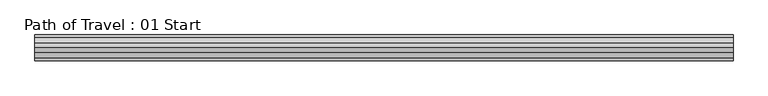
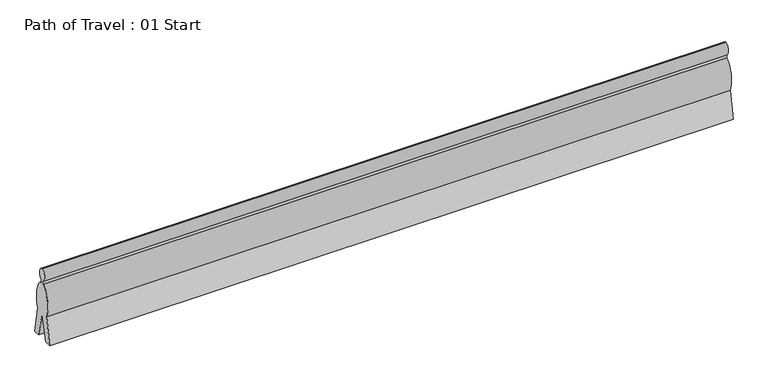
"""IFC4 building model written with IfcOpenShell, lengths in millimetres: proxy geometry, Path of Travel : 01 Start."""

from ifc_helpers import new_model, si_unit, point, frame, origin, place, context, project, spatial, ellipse_curve, trimmed, source, transform, mapped, element, save
from ifc_brep_helpers import plane_surface, extruded_surface, advanced_brep


def path_of_travel_01_start_60fd2745(model_context):
    return source(origin(), model_context, "Body", "AdvancedBrep", [
        advanced_brep(
        [(227.5554837, 0.0, 1727.2), (227.5554837, 42.9018657, 1436.6534209), (227.5554837, 42.9018657, 1363.4763406), (227.5554837, 184.1186263, 643.4144547), (227.5554837, 297.5699544, 0.0), (227.5554837, 145.6574193, 0.0), (227.5554837, 0.0, 584.2), (227.5554837, -145.6574193, 0.0), (227.5554837, -297.5699544, 0.0), (227.5554837, -184.1186263, 643.4144547), (227.5554837, -42.9018657, 1363.4763406), (227.5554837, -42.9018657, 1436.6534209), (16229.5554837, 0.0, 1727.2), (16229.5554837, -42.9018657, 1436.6534209), (16229.5554837, -42.9018657, 1363.4763406), (16229.5554837, -184.1186263, 643.4144547), (16229.5554837, -297.5699544, 0.0), (16229.5554837, -145.6574193, 0.0), (16229.5554837, 0.0, 584.2), (16229.5554837, 145.6574193, 0.0), (16229.5554837, 297.5699544, 0.0), (16229.5554837, 184.1186263, 643.4144547), (16229.5554837, 42.9018657, 1363.4763406), (16229.5554837, 42.9018657, 1436.6534209)],
        [
            (0, 1, ellipse_curve(frame((227.5554837, 0.0, 1574.8), z_axis=(-1.0, 0.0, 0.0), x_axis=(0.0, 0.0, 1.0)), 152.4, 101.6)),
            (1, 2),
            (2, 3, ellipse_curve(frame((227.5554837, 0.0, 914.4), z_axis=(-1.0, 0.0, 0.0), x_axis=(0.0, 0.0, -1.0)), 457.2, 228.6)),
            (3, 4),
            (4, 5),
            (5, 6),
            (6, 7),
            (7, 8),
            (8, 9),
            (9, 10, ellipse_curve(frame((227.5554837, 0.0, 914.4), z_axis=(-1.0, 0.0, 0.0), x_axis=(0.0, 0.0, -1.0)), 457.2, 228.6)),
            (10, 11),
            (11, 0, ellipse_curve(frame((227.5554837, 0.0, 1574.8), z_axis=(-1.0, 0.0, 0.0), x_axis=(0.0, 0.0, 1.0)), 152.4, 101.6)),
            (12, 13, ellipse_curve(frame((16229.5554837, 0.0, 1574.8), z_axis=(1.0, 0.0, 0.0), x_axis=(0.0, 0.0, 1.0)), 152.4, 101.6)),
            (13, 14),
            (14, 15, ellipse_curve(frame((16229.5554837, 0.0, 914.4), z_axis=(1.0, 0.0, 0.0), x_axis=(0.0, 0.0, -1.0)), 457.2, 228.6)),
            (15, 16),
            (16, 17),
            (17, 18),
            (18, 19),
            (19, 20),
            (20, 21),
            (21, 22, ellipse_curve(frame((16229.5554837, 0.0, 914.4), z_axis=(1.0, 0.0, 0.0), x_axis=(0.0, 0.0, -1.0)), 457.2, 228.6)),
            (22, 23),
            (23, 12, ellipse_curve(frame((16229.5554837, 0.0, 1574.8), z_axis=(1.0, 0.0, 0.0), x_axis=(0.0, 0.0, 1.0)), 152.4, 101.6)),
            (0, 12),
            (23, 1),
            (22, 2),
            (21, 3),
            (20, 4),
            (19, 5),
            (18, 6),
            (17, 7),
            (16, 8),
            (15, 9),
            (14, 10),
            (13, 11),
        ],
        [
            plane_surface(frame((227.5554837, 0.0, 0.0), z_axis=(-1.0, 0.0, 0.0), x_axis=(0.0, 0.0, 1.0))),
            plane_surface(frame((16229.5554837, 0.0, 0.0), z_axis=(1.0, 0.0, 0.0), x_axis=(0.0, 0.0, 1.0))),
            extruded_surface(trimmed(ellipse_curve(frame((16229.5554837, 0.0, 1574.8), z_axis=(-1.0, 0.0, 0.0), x_axis=(0.0, 0.0, 1.0)), 152.4, 101.6), [point((16229.5554837, 0.0, 1727.2))], [point((16229.5554837, 42.9018657, 1436.6534209))], True, "CARTESIAN"), (-16002.0, 0.0, 0.0), 16002.0),
            plane_surface(frame((227.5554837, 42.9018657, 1436.6534209), z_axis=(0.0, 1.0, 0.0), x_axis=(1.0, 0.0, 0.0))),
            extruded_surface(trimmed(ellipse_curve(frame((16229.5554837, 0.0, 914.4), z_axis=(-1.0, 0.0, 0.0), x_axis=(0.0, 0.0, -1.0)), 457.2, 228.6), [point((16229.5554837, 42.9018657, 1363.4763406))], [point((16229.5554837, 184.1186263, 643.4144547))], True, "CARTESIAN"), (-16002.0, 0.0, 0.0), 16002.0),
            plane_surface(frame((227.5554837, 184.1186263, 643.4144547), z_axis=(0.0, 0.9848077530122078, 0.17364817766693205), x_axis=(1.0, 0.0, 0.0))),
            plane_surface(frame((227.5554837, 297.5699544, 0.0), z_axis=(0.0, 0.0, -1.0), x_axis=(1.0, 0.0, 0.0))),
            plane_surface(frame((227.5554837, 145.6574193, 0.0), z_axis=(0.0, -0.9702957262760199, -0.2419218955995739), x_axis=(1.0, 0.0, 0.0))),
            plane_surface(frame((227.5554837, 0.0, 584.2), z_axis=(0.0, 0.9702957262759961, -0.24192189559966923), x_axis=(1.0, 0.0, 0.0))),
            plane_surface(frame((227.5554837, -145.6574193, 0.0), z_axis=(0.0, 0.0, -1.0), x_axis=(1.0, 0.0, 0.0))),
            plane_surface(frame((227.5554837, -297.5699544, 0.0), z_axis=(0.0, -0.984807753012208, 0.17364817766693066), x_axis=(1.0, 0.0, 0.0))),
            extruded_surface(trimmed(ellipse_curve(frame((16229.5554837, 0.0, 914.4), z_axis=(-1.0, 0.0, 0.0), x_axis=(0.0, 0.0, -1.0)), 457.2, 228.6), [point((16229.5554837, -184.1186263, 643.4144547))], [point((16229.5554837, -42.9018657, 1363.4763406))], True, "CARTESIAN"), (-16002.0, 0.0, 0.0), 16002.0),
            plane_surface(frame((227.5554837, -42.9018657, 1363.4763406), z_axis=(0.0, -1.0, 0.0), x_axis=(1.0, 0.0, 0.0))),
            extruded_surface(trimmed(ellipse_curve(frame((16229.5554837, 0.0, 1574.8), z_axis=(-1.0, 0.0, 0.0), x_axis=(0.0, 0.0, 1.0)), 152.4, 101.6), [point((16229.5554837, -42.9018657, 1436.6534209))], [point((16229.5554837, 0.0, 1727.2))], True, "CARTESIAN"), (-16002.0, 0.0, 0.0), 16002.0),
        ],
        [
            (0, [[1, 2, 3, 4, 5, 6, 7, 8, 9, 10, 11, 12]]),
            (1, [[13, 14, 15, 16, 17, 18, 19, 20, 21, 22, 23, 24]]),
            (2, [[-1, 25, -24, 26]]),
            (3, [[-2, -26, -23, 27]]),
            (4, [[-3, -27, -22, 28]]),
            (5, [[-4, -28, -21, 29]]),
            (6, [[-5, -29, -20, 30]]),
            (7, [[-6, -30, -19, 31]]),
            (8, [[-7, -31, -18, 32]]),
            (9, [[-8, -32, -17, 33]]),
            (10, [[-9, -33, -16, 34]]),
            (11, [[-10, -34, -15, 35]]),
            (12, [[-11, -35, -14, 36]]),
            (13, [[-12, -36, -13, -25]]),
        ],
    ),
    ])


if __name__ == "__main__":
    model = new_model("IFC4")
    model_context = context("Model", 3, world=origin())
    ifc_project = project(units=[si_unit("LENGTHUNIT", "METRE", prefix="MILLI")], contexts=[model_context])
    site = spatial("IfcSite", under=ifc_project)
    building = spatial("IfcBuilding", under=site)
    placement = place(None, origin())
    path_of_travel_01_start_shape = path_of_travel_01_start_60fd2745(model_context)
    element("IfcBuildingElementProxy", 1, Name="Path of Travel : 01 Start", ObjectType="Path of Travel : 01 Start", at=placement, inside=building, context=model_context, shape_type="MappedRepresentation", body=[
        mapped(path_of_travel_01_start_shape, transform((0.0, 0.0, 0.0), x_axis=(1.0, 0.0, 0.0), y_axis=(0.0, 1.0, 0.0), z_axis=(0.0, 0.0, 1.0))),
    ])
    save(model, "model.ifc")

# Revit data of these elements
# Type "Path of Travel : 01 Start"
#   Path of Egress [instance default] = 4' - 0"
#   built-in parameter 1001306 [instance default] = 4 (stored number, unit not read)
#   Dot at Start = yes
#   Arrow in Middle = yes
#   Arrow at End = no
#   Egress Path = none
# Element 1 (IfcBuildingElementProxy, "Path of Travel : 01 Start")
#   Path of Egress = 52' - 6"
#   built-in parameter 1001306 = 52.5 (stored number, unit not read)
#   Materials on its faces: "Egress Path Solid"
# Materials
#   "Egress Path Solid": class "Unassigned", colour RGB 255 128 64, transparency 0.75, Comments = "Rendering appearance not upgraded "
